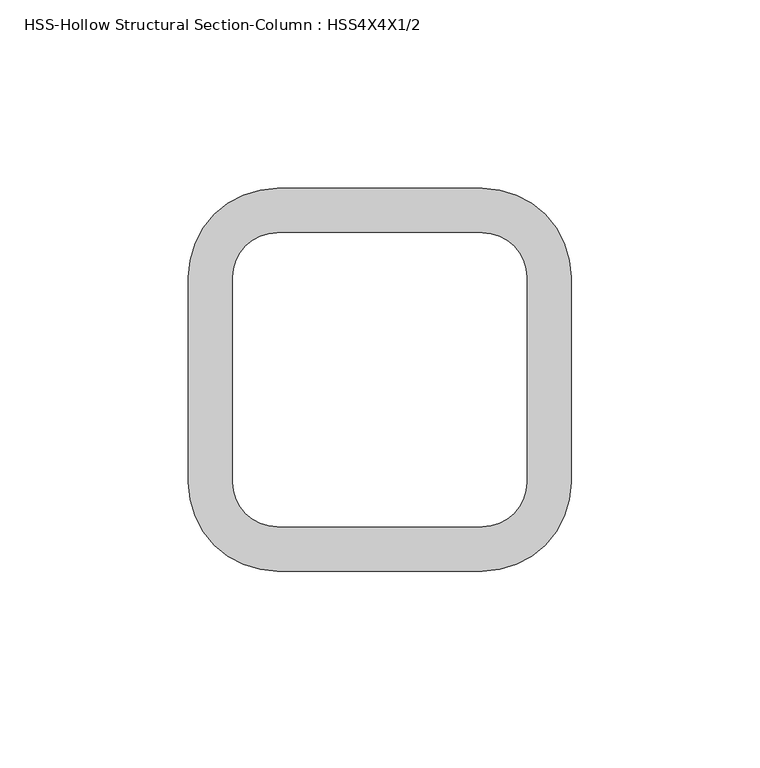
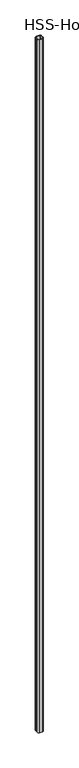
"""IFC4 building model written with IfcOpenShell, lengths in millimetres: column geometry, HSS-Hollow Structural Section-Column : HSS4X4X1/2."""

from ifc_helpers import new_model, si_unit, point, frame, frame_2d, origin, place, context, project, spatial, polyline, circle_curve, trimmed, segment, composite_curve, outline, extrude, source, transform, mapped, element, save


def hss_hollow_structural_section_column_hss4x4x1_2_ea61a488(model_context):
    return source(origin(), model_context, "Body", "SweptSolid", [
        extrude(outline(composite_curve([segment(trimmed(circle_curve(frame_2d((27.178, 27.178)), 23.622), [point((27.178, 50.8))], [point((50.8, 27.178))], False, "CARTESIAN"), True, "CONTINUOUS"), segment(polyline([(50.8, 27.178), (50.8, -27.178)]), True, "CONTINUOUS"), segment(trimmed(circle_curve(frame_2d((27.178, -27.178)), 23.622), [point((50.8, -27.178))], [point((27.178, -50.8))], False, "CARTESIAN"), True, "CONTINUOUS"), segment(polyline([(27.178, -50.8), (-27.178, -50.8)]), True, "CONTINUOUS"), segment(trimmed(circle_curve(frame_2d((-27.178, -27.178)), 23.622), [point((-27.178, -50.8))], [point((-50.8, -27.178))], False, "CARTESIAN"), True, "CONTINUOUS"), segment(polyline([(-50.8, -27.178), (-50.8, 27.178)]), True, "CONTINUOUS"), segment(trimmed(circle_curve(frame_2d((-27.178, 27.178)), 23.622), [point((-50.8, 27.178))], [point((-27.178, 50.8))], False, "CARTESIAN"), True, "CONTINUOUS"), segment(polyline([(-27.178, 50.8), (27.178, 50.8)]), True, "CONTINUOUS")], self_intersect=False), holes=[composite_curve([segment(polyline([(27.178, 38.989), (-27.178, 38.989)]), True, "CONTINUOUS"), segment(trimmed(circle_curve(frame_2d((-27.178, 27.178)), 11.811), [point((-27.178, 38.989))], [point((-38.989, 27.178))], True, "CARTESIAN"), True, "CONTINUOUS"), segment(polyline([(-38.989, 27.178), (-38.989, -27.178)]), True, "CONTINUOUS"), segment(trimmed(circle_curve(frame_2d((-27.178, -27.178)), 11.811), [point((-38.989, -27.178))], [point((-27.178, -38.989))], True, "CARTESIAN"), True, "CONTINUOUS"), segment(polyline([(-27.178, -38.989), (27.178, -38.989)]), True, "CONTINUOUS"), segment(trimmed(circle_curve(frame_2d((27.178, -27.178)), 11.811), [point((27.178, -38.989))], [point((38.989, -27.178))], True, "CARTESIAN"), True, "CONTINUOUS"), segment(polyline([(38.989, -27.178), (38.989, 27.178)]), True, "CONTINUOUS"), segment(trimmed(circle_curve(frame_2d((27.178, 27.178)), 11.811), [point((38.989, 27.178))], [point((27.178, 38.989))], True, "CARTESIAN"), True, "CONTINUOUS")], self_intersect=False)]), frame((0.0, 0.0, -609.6), z_axis=(0.0, 0.0, 1.0), x_axis=(1.0, 0.0, 0.0)), (0.0, 0.0, 1.0), 12903.2),
    ])


if __name__ == "__main__":
    model = new_model("IFC4")
    model_context = context("Model", 3, world=origin())
    ifc_project = project(units=[si_unit("LENGTHUNIT", "METRE", prefix="MILLI")], contexts=[model_context])
    site = spatial("IfcSite", under=ifc_project)
    building = spatial("IfcBuilding", under=site)
    placement = place(None, origin())
    hss_hollow_structural_section_column_hss4x4x1_2_shape = hss_hollow_structural_section_column_hss4x4x1_2_ea61a488(model_context)
    element("IfcColumn", 1, ObjectType="HSS-Hollow Structural Section-Column : HSS4X4X1/2", at=placement, inside=building, context=model_context, shape_type="MappedRepresentation", body=[
        mapped(hss_hollow_structural_section_column_hss4x4x1_2_shape, transform((0.0, 0.0, 0.0), x_axis=(1.0, 0.0, 0.0), y_axis=(0.0, 1.0, 0.0), z_axis=(0.0, 0.0, 1.0))),
    ])
    save(model, "model.ifc")

# Revit data of these elements
# Type "HSS-Hollow Structural Section-Column : HSS4X4X1/2"
#   Assembly Code = "B10"
#   Shape = "Square"
#   W = 21.5
#   Ht = 0' - 4"
#   b = 0' - 4"
#   kr = 0' - 0.93"
#   t = 0' - 0.465"
#   A = 0.0418056 SF
#   Structural Material [instance default] = Steel ASTM A500, Grade B, Rectangular and Square
# Element 1 (IfcColumn, "HSS-Hollow Structural Section-Column : HSS4X4X1/2")
#   Materials on its faces: "Steel ASTM A500, Grade B, Rectangular and Square"
# Materials
#   "Steel ASTM A500, Grade B, Rectangular and Square": class "Metal", colour RGB 199 199 199, transparency 0, Description = "Carbon steel", Cost = 0
